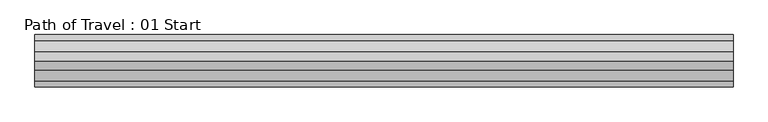
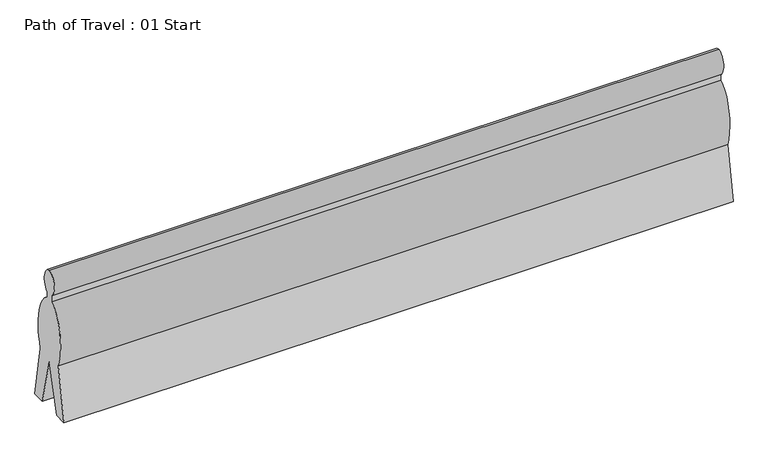
"""IFC4 building model written with IfcOpenShell, lengths in millimetres: proxy geometry, Path of Travel : 01 Start."""

from ifc_helpers import new_model, si_unit, point, frame, origin, place, context, project, spatial, ellipse_curve, trimmed, source, transform, mapped, element, save
from ifc_brep_helpers import plane_surface, extruded_surface, advanced_brep


def path_of_travel_01_start_bf55958a(model_context):
    return source(origin(), model_context, "Body", "AdvancedBrep", [
        advanced_brep(
        [(227.5554837, 0.0, 1727.2), (227.5554837, 42.9018657, 1436.6534209), (227.5554837, 42.9018657, 1363.4763406), (227.5554837, 184.1186263, 643.4144547), (227.5554837, 297.5699544, 0.0), (227.5554837, 145.6574193, 0.0), (227.5554837, 0.0, 584.2), (227.5554837, -145.6574193, 0.0), (227.5554837, -297.5699544, 0.0), (227.5554837, -184.1186263, 643.4144547), (227.5554837, -42.9018657, 1363.4763406), (227.5554837, -42.9018657, 1436.6534209), (8152.3554837, 0.0, 1727.2), (8152.3554837, -42.9018657, 1436.6534209), (8152.3554837, -42.9018657, 1363.4763406), (8152.3554837, -184.1186263, 643.4144547), (8152.3554837, -297.5699544, 0.0), (8152.3554837, -145.6574193, 0.0), (8152.3554837, 0.0, 584.2), (8152.3554837, 145.6574193, 0.0), (8152.3554837, 297.5699544, 0.0), (8152.3554837, 184.1186263, 643.4144547), (8152.3554837, 42.9018657, 1363.4763406), (8152.3554837, 42.9018657, 1436.6534209)],
        [
            (0, 1, ellipse_curve(frame((227.5554837, 0.0, 1574.8), z_axis=(-1.0, 0.0, 0.0), x_axis=(0.0, 0.0, 1.0)), 152.4, 101.6)),
            (1, 2),
            (2, 3, ellipse_curve(frame((227.5554837, 0.0, 914.4), z_axis=(-1.0, 0.0, 0.0), x_axis=(0.0, 0.0, -1.0)), 457.2, 228.6)),
            (3, 4),
            (4, 5),
            (5, 6),
            (6, 7),
            (7, 8),
            (8, 9),
            (9, 10, ellipse_curve(frame((227.5554837, 0.0, 914.4), z_axis=(-1.0, 0.0, 0.0), x_axis=(0.0, 0.0, -1.0)), 457.2, 228.6)),
            (10, 11),
            (11, 0, ellipse_curve(frame((227.5554837, 0.0, 1574.8), z_axis=(-1.0, 0.0, 0.0), x_axis=(0.0, 0.0, 1.0)), 152.4, 101.6)),
            (12, 13, ellipse_curve(frame((8152.3554837, 0.0, 1574.8), z_axis=(1.0, 0.0, 0.0), x_axis=(0.0, 0.0, 1.0)), 152.4, 101.6)),
            (13, 14),
            (14, 15, ellipse_curve(frame((8152.3554837, 0.0, 914.4), z_axis=(1.0, 0.0, 0.0), x_axis=(0.0, 0.0, -1.0)), 457.2, 228.6)),
            (15, 16),
            (16, 17),
            (17, 18),
            (18, 19),
            (19, 20),
            (20, 21),
            (21, 22, ellipse_curve(frame((8152.3554837, 0.0, 914.4), z_axis=(1.0, 0.0, 0.0), x_axis=(0.0, 0.0, -1.0)), 457.2, 228.6)),
            (22, 23),
            (23, 12, ellipse_curve(frame((8152.3554837, 0.0, 1574.8), z_axis=(1.0, 0.0, 0.0), x_axis=(0.0, 0.0, 1.0)), 152.4, 101.6)),
            (0, 12),
            (23, 1),
            (22, 2),
            (21, 3),
            (20, 4),
            (19, 5),
            (18, 6),
            (17, 7),
            (16, 8),
            (15, 9),
            (14, 10),
            (13, 11),
        ],
        [
            plane_surface(frame((227.5554837, 0.0, 0.0), z_axis=(-1.0, 0.0, 0.0), x_axis=(0.0, 0.0, 1.0))),
            plane_surface(frame((8152.3554837, 0.0, 0.0), z_axis=(1.0, 0.0, 0.0), x_axis=(0.0, 0.0, 1.0))),
            extruded_surface(trimmed(ellipse_curve(frame((8152.3554837, 0.0, 1574.8), z_axis=(-1.0, 0.0, 0.0), x_axis=(0.0, 0.0, 1.0)), 152.4, 101.6), [point((8152.3554837, 0.0, 1727.2))], [point((8152.3554837, 42.9018657, 1436.6534209))], True, "CARTESIAN"), (-7924.8, 0.0, 0.0), 7924.8),
            plane_surface(frame((227.5554837, 42.9018657, 1436.6534209), z_axis=(0.0, 1.0, 0.0), x_axis=(1.0, 0.0, 0.0))),
            extruded_surface(trimmed(ellipse_curve(frame((8152.3554837, 0.0, 914.4), z_axis=(-1.0, 0.0, 0.0), x_axis=(0.0, 0.0, -1.0)), 457.2, 228.6), [point((8152.3554837, 42.9018657, 1363.4763406))], [point((8152.3554837, 184.1186263, 643.4144547))], True, "CARTESIAN"), (-7924.8, 0.0, 0.0), 7924.8),
            plane_surface(frame((227.5554837, 184.1186263, 643.4144547), z_axis=(0.0, 0.9848077530122078, 0.17364817766693205), x_axis=(1.0, 0.0, 0.0))),
            plane_surface(frame((227.5554837, 297.5699544, 0.0), z_axis=(0.0, 0.0, -1.0), x_axis=(1.0, 0.0, 0.0))),
            plane_surface(frame((227.5554837, 145.6574193, 0.0), z_axis=(0.0, -0.9702957262760199, -0.2419218955995739), x_axis=(1.0, 0.0, 0.0))),
            plane_surface(frame((227.5554837, 0.0, 584.2), z_axis=(0.0, 0.9702957262759961, -0.24192189559966923), x_axis=(1.0, 0.0, 0.0))),
            plane_surface(frame((227.5554837, -145.6574193, 0.0), z_axis=(0.0, 0.0, -1.0), x_axis=(1.0, 0.0, 0.0))),
            plane_surface(frame((227.5554837, -297.5699544, 0.0), z_axis=(0.0, -0.984807753012208, 0.17364817766693066), x_axis=(1.0, 0.0, 0.0))),
            extruded_surface(trimmed(ellipse_curve(frame((8152.3554837, 0.0, 914.4), z_axis=(-1.0, 0.0, 0.0), x_axis=(0.0, 0.0, -1.0)), 457.2, 228.6), [point((8152.3554837, -184.1186263, 643.4144547))], [point((8152.3554837, -42.9018657, 1363.4763406))], True, "CARTESIAN"), (-7924.8, 0.0, 0.0), 7924.8),
            plane_surface(frame((227.5554837, -42.9018657, 1363.4763406), z_axis=(0.0, -1.0, 0.0), x_axis=(1.0, 0.0, 0.0))),
            extruded_surface(trimmed(ellipse_curve(frame((8152.3554837, 0.0, 1574.8), z_axis=(-1.0, 0.0, 0.0), x_axis=(0.0, 0.0, 1.0)), 152.4, 101.6), [point((8152.3554837, -42.9018657, 1436.6534209))], [point((8152.3554837, 0.0, 1727.2))], True, "CARTESIAN"), (-7924.8, 0.0, 0.0), 7924.8),
        ],
        [
            (0, [[1, 2, 3, 4, 5, 6, 7, 8, 9, 10, 11, 12]]),
            (1, [[13, 14, 15, 16, 17, 18, 19, 20, 21, 22, 23, 24]]),
            (2, [[-1, 25, -24, 26]]),
            (3, [[-2, -26, -23, 27]]),
            (4, [[-3, -27, -22, 28]]),
            (5, [[-4, -28, -21, 29]]),
            (6, [[-5, -29, -20, 30]]),
            (7, [[-6, -30, -19, 31]]),
            (8, [[-7, -31, -18, 32]]),
            (9, [[-8, -32, -17, 33]]),
            (10, [[-9, -33, -16, 34]]),
            (11, [[-10, -34, -15, 35]]),
            (12, [[-11, -35, -14, 36]]),
            (13, [[-12, -36, -13, -25]]),
        ],
    ),
    ])


if __name__ == "__main__":
    model = new_model("IFC4")
    model_context = context("Model", 3, world=origin())
    ifc_project = project(units=[si_unit("LENGTHUNIT", "METRE", prefix="MILLI")], contexts=[model_context])
    site = spatial("IfcSite", under=ifc_project)
    building = spatial("IfcBuilding", under=site)
    placement = place(None, origin())
    path_of_travel_01_start_shape = path_of_travel_01_start_bf55958a(model_context)
    element("IfcBuildingElementProxy", 1, Name="Path of Travel : 01 Start", ObjectType="Path of Travel : 01 Start", at=placement, inside=building, context=model_context, shape_type="MappedRepresentation", body=[
        mapped(path_of_travel_01_start_shape, transform((0.0, 0.0, 0.0), x_axis=(1.0, 0.0, 0.0), y_axis=(0.0, 1.0, 0.0), z_axis=(0.0, 0.0, 1.0))),
    ])
    save(model, "model.ifc")

# Revit data of these elements
# Type "Path of Travel : 01 Start"
#   Path of Egress [instance default] = 4' - 0"
#   built-in parameter 1001306 [instance default] = 4 (stored number, unit not read)
#   Dot at Start = yes
#   Arrow in Middle = yes
#   Arrow at End = no
#   Egress Path = none
# Element 1 (IfcBuildingElementProxy, "Path of Travel : 01 Start")
#   Path of Egress = 26' - 0"
#   built-in parameter 1001306 = 26 (stored number, unit not read)
#   Materials on its faces: "Egress Path Solid"
# Materials
#   "Egress Path Solid": class "Unassigned", colour RGB 255 128 64, transparency 0.75, Comments = "Rendering appearance not upgraded "
